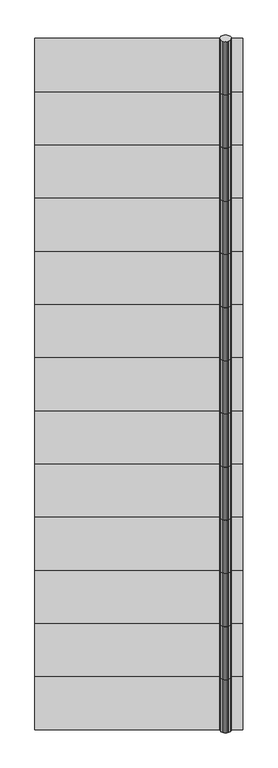
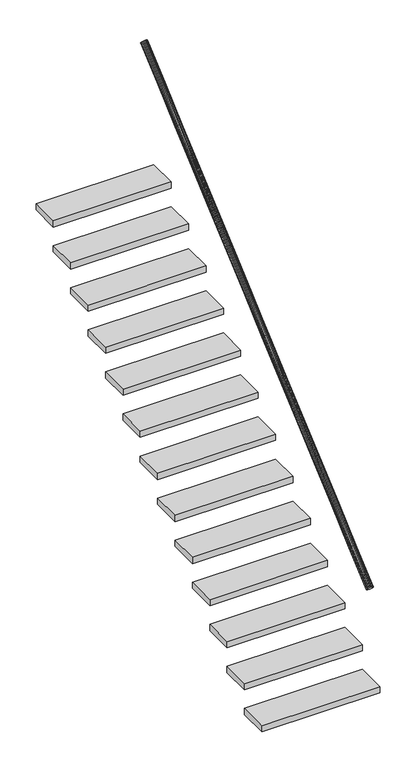
"""IFC4 building model written with IfcOpenShell, lengths in millimetres: stair geometry, 0_3d."""

from ifc_helpers import new_model, si_unit, frame, origin, origin_with_axes, place, context, project, spatial, polyline, outline, extrude, source, transform, mapped, element, save


def stair_800c35a0(model_context):
    return source(origin(), model_context, "Body", "SweptSolid", [
        extrude(outline(polyline([(900.0, 1165.003504), (0.0, 1165.003504), (0.0, 1395.003504), (900.0, 1395.003504), (900.0, 1165.003504)])), frame((0.0, 0.0, 1000.0), z_axis=(0.0, 0.0, 1.0), x_axis=(1.0, 0.0, 0.0)), (0.0, 0.0, 1.0), 50.0),
        extrude(outline(polyline([(900.0, 245.003504), (0.0, 245.003504), (0.0, 475.003504), (900.0, 475.003504), (900.0, 245.003504)])), frame((0.0, 0.0, 200.0), z_axis=(0.0, 0.0, 1.0), x_axis=(1.0, 0.0, 0.0)), (0.0, 0.0, 1.0), 50.0),
        extrude(outline(polyline([(1.2235871, -7.0656631), (0.0, 0.0), (1.2235871, 7.065663), (4.7745751, 13.4396897), (10.3053687, 18.4981459), (17.2745751, 21.7458748), (25.0, 22.8649659), (32.7254249, 21.7458748), (39.6946313, 18.4981459), (45.2254249, 13.4396897), (48.7764129, 7.065663), (50.0, 0.0), (48.7764129, -7.0656631), (45.2254249, -13.4396898), (39.6946313, -18.498146), (32.7254249, -21.7458748), (25.0, -22.864966), (17.2745751, -21.7458748), (10.3053687, -18.498146), (4.7745751, -13.4396898), (1.2235871, -7.0656631)])), frame((800.0, 1165.003504, 1869.5592366), z_axis=(0.0, 0.7546055221634054, 0.656178714924901), x_axis=(1.0, 0.0, 0.0)), (0.0, 0.0, 1.0), 304.7950131),
        extrude(outline(polyline([(1.2235871, -7.0656631), (0.0, 0.0), (1.2235871, 7.065663), (4.7745751, 13.4396897), (10.3053687, 18.4981459), (17.2745751, 21.7458748), (25.0, 22.8649659), (32.7254249, 21.7458748), (39.6946313, 18.4981459), (45.2254249, 13.4396897), (48.7764129, 7.065663), (50.0, 0.0), (48.7764129, -7.0656631), (45.2254249, -13.4396898), (39.6946313, -18.498146), (32.7254249, -21.7458748), (25.0, -22.864966), (17.2745751, -21.7458748), (10.3053687, -18.498146), (4.7745751, -13.4396898), (1.2235871, -7.0656631)])), frame((800.0, 475.003504, 1269.5592366), z_axis=(0.0, 0.7546055221634524, 0.6561787149248467), x_axis=(1.0, 0.0, 0.0)), (0.0, 0.0, 1.0), 304.7950131),
        extrude(outline(polyline([(1.2235871, -7.0656631), (0.0, 0.0), (1.2235871, 7.065663), (4.7745751, 13.4396897), (10.3053687, 18.4981459), (17.2745751, 21.7458748), (25.0, 22.8649659), (32.7254249, 21.7458748), (39.6946313, 18.4981459), (45.2254249, 13.4396897), (48.7764129, 7.065663), (50.0, 0.0), (48.7764129, -7.0656631), (45.2254249, -13.4396898), (39.6946313, -18.498146), (32.7254249, -21.7458748), (25.0, -22.864966), (17.2745751, -21.7458748), (10.3053687, -18.498146), (4.7745751, -13.4396898), (1.2235871, -7.0656631)])), frame((800.0, 2315.003504, 2869.5592366), z_axis=(0.0, 0.7546055221634114, 0.656178714924894), x_axis=(1.0, 0.0, 0.0)), (0.0, 0.0, 1.0), 304.7950131),
        extrude(outline(polyline([(1.2235871, -7.0656631), (0.0, 0.0), (1.2235871, 7.065663), (4.7745751, 13.4396897), (10.3053687, 18.4981459), (17.2745751, 21.7458748), (25.0, 22.8649659), (32.7254249, 21.7458748), (39.6946313, 18.4981459), (45.2254249, 13.4396897), (48.7764129, 7.065663), (50.0, 0.0), (48.7764129, -7.0656631), (45.2254249, -13.4396898), (39.6946313, -18.498146), (32.7254249, -21.7458748), (25.0, -22.864966), (17.2745751, -21.7458748), (10.3053687, -18.498146), (4.7745751, -13.4396898), (1.2235871, -7.0656631)])), frame((800.0, 705.003504, 1469.5592366), z_axis=(0.0, 0.7546055221634539, 0.656178714924845), x_axis=(1.0, 0.0, 0.0)), (0.0, 0.0, 1.0), 304.7950131),
        extrude(outline(polyline([(900.0, 2545.003504), (0.0, 2545.003504), (0.0, 2775.003504), (900.0, 2775.003504), (900.0, 2545.003504)])), frame((0.0, 0.0, 2200.0), z_axis=(0.0, 0.0, 1.0), x_axis=(1.0, 0.0, 0.0)), (0.0, 0.0, 1.0), 50.0),
        extrude(outline(polyline([(1.2235871, -7.0656631), (0.0, 0.0), (1.2235871, 7.065663), (4.7745751, 13.4396897), (10.3053687, 18.4981459), (17.2745751, 21.7458748), (25.0, 22.8649659), (32.7254249, 21.7458748), (39.6946313, 18.4981459), (45.2254249, 13.4396897), (48.7764129, 7.065663), (50.0, 0.0), (48.7764129, -7.0656631), (45.2254249, -13.4396898), (39.6946313, -18.498146), (32.7254249, -21.7458748), (25.0, -22.864966), (17.2745751, -21.7458748), (10.3053687, -18.498146), (4.7745751, -13.4396898), (1.2235871, -7.0656631)])), frame((800.0, 245.003504, 1069.5592366), z_axis=(0.0, 0.7546055221634513, 0.656178714924848), x_axis=(1.0, 0.0, 0.0)), (0.0, 0.0, 1.0), 304.7950131),
        extrude(outline(polyline([(1.2235871, -7.0656631), (0.0, 0.0), (1.2235871, 7.065663), (4.7745751, 13.4396897), (10.3053687, 18.4981459), (17.2745751, 21.7458748), (25.0, 22.8649659), (32.7254249, 21.7458748), (39.6946313, 18.4981459), (45.2254249, 13.4396897), (48.7764129, 7.065663), (50.0, 0.0), (48.7764129, -7.0656631), (45.2254249, -13.4396898), (39.6946313, -18.498146), (32.7254249, -21.7458748), (25.0, -22.864966), (17.2745751, -21.7458748), (10.3053687, -18.498146), (4.7745751, -13.4396898), (1.2235871, -7.0656631)])), frame((800.0, 2775.003504, 3269.5592366), z_axis=(0.0, 0.7546055221634004, 0.6561787149249065), x_axis=(1.0, 0.0, 0.0)), (0.0, 0.0, 1.0), 304.7950131),
        extrude(outline(polyline([(1.2235871, -7.0656631), (0.0, 0.0), (1.2235871, 7.065663), (4.7745751, 13.4396897), (10.3053687, 18.4981459), (17.2745751, 21.7458748), (25.0, 22.8649659), (32.7254249, 21.7458748), (39.6946313, 18.4981459), (45.2254249, 13.4396897), (48.7764129, 7.065663), (50.0, 0.0), (48.7764129, -7.0656631), (45.2254249, -13.4396898), (39.6946313, -18.498146), (32.7254249, -21.7458748), (25.0, -22.864966), (17.2745751, -21.7458748), (10.3053687, -18.498146), (4.7745751, -13.4396898), (1.2235871, -7.0656631)])), frame((800.0, 15.003504, 869.5592366), z_axis=(0.0, 0.7546055221634687, 0.6561787149248283), x_axis=(1.0, 0.0, 0.0)), (0.0, 0.0, 1.0), 304.7950131),
        extrude(outline(polyline([(900.0, 475.003504), (0.0, 475.003504), (0.0, 705.003504), (900.0, 705.003504), (900.0, 475.003504)])), frame((0.0, 0.0, 400.0), z_axis=(0.0, 0.0, 1.0), x_axis=(1.0, 0.0, 0.0)), (0.0, 0.0, 1.0), 50.0),
        extrude(outline(polyline([(1.2235871, -7.0656631), (0.0, 0.0), (1.2235871, 7.065663), (4.7745751, 13.4396897), (10.3053687, 18.4981459), (17.2745751, 21.7458748), (25.0, 22.8649659), (32.7254249, 21.7458748), (39.6946313, 18.4981459), (45.2254249, 13.4396897), (48.7764129, 7.065663), (50.0, 0.0), (48.7764129, -7.0656631), (45.2254249, -13.4396898), (39.6946313, -18.498146), (32.7254249, -21.7458748), (25.0, -22.864966), (17.2745751, -21.7458748), (10.3053687, -18.498146), (4.7745751, -13.4396898), (1.2235871, -7.0656631)])), frame((800.0, 1625.003504, 2269.5592366), z_axis=(0.0, 0.7546055221634052, 0.6561787149249012), x_axis=(1.0, 0.0, 0.0)), (0.0, 0.0, 1.0), 304.7950131),
        extrude(outline(polyline([(1.2235871, -7.0656631), (0.0, 0.0), (1.2235871, 7.065663), (4.7745751, 13.4396897), (10.3053687, 18.4981459), (17.2745751, 21.7458748), (25.0, 22.8649659), (32.7254249, 21.7458748), (39.6946313, 18.4981459), (45.2254249, 13.4396897), (48.7764129, 7.065663), (50.0, 0.0), (48.7764129, -7.0656631), (45.2254249, -13.4396898), (39.6946313, -18.498146), (32.7254249, -21.7458748), (25.0, -22.864966), (17.2745751, -21.7458748), (10.3053687, -18.498146), (4.7745751, -13.4396898), (1.2235871, -7.0656631)])), frame((800.0, 2545.003504, 3069.5592366), z_axis=(0.0, 0.7546055221634068, 0.6561787149248993), x_axis=(1.0, 0.0, 0.0)), (0.0, 0.0, 1.0), 304.7950131),
        extrude(outline(polyline([(900.0, 1395.003504), (0.0, 1395.003504), (0.0, 1625.003504), (900.0, 1625.003504), (900.0, 1395.003504)])), frame((0.0, 0.0, 1200.0), z_axis=(0.0, 0.0, 1.0), x_axis=(1.0, 0.0, 0.0)), (0.0, 0.0, 1.0), 50.0),
        extrude(outline(polyline([(900.0, 1855.003504), (0.0, 1855.003504), (0.0, 2085.003504), (900.0, 2085.003504), (900.0, 1855.003504)])), frame((0.0, 0.0, 1600.0), z_axis=(0.0, 0.0, 1.0), x_axis=(1.0, 0.0, 0.0)), (0.0, 0.0, 1.0), 50.0),
        extrude(outline(polyline([(1.2235871, -7.0656631), (0.0, 0.0), (1.2235871, 7.065663), (4.7745751, 13.4396897), (10.3053687, 18.4981459), (17.2745751, 21.7458748), (25.0, 22.8649659), (32.7254249, 21.7458748), (39.6946313, 18.4981459), (45.2254249, 13.4396897), (48.7764129, 7.065663), (50.0, 0.0), (48.7764129, -7.0656631), (45.2254249, -13.4396898), (39.6946313, -18.498146), (32.7254249, -21.7458748), (25.0, -22.864966), (17.2745751, -21.7458748), (10.3053687, -18.498146), (4.7745751, -13.4396898), (1.2235871, -7.0656631)])), frame((800.0, 1395.003504, 2069.5592366), z_axis=(0.0, 0.7546055221634034, 0.6561787149249032), x_axis=(1.0, 0.0, 0.0)), (0.0, 0.0, 1.0), 304.7950131),
        extrude(outline(polyline([(900.0, 935.003504), (0.0, 935.003504), (0.0, 1165.003504), (900.0, 1165.003504), (900.0, 935.003504)])), frame((0.0, 0.0, 800.0), z_axis=(0.0, 0.0, 1.0), x_axis=(1.0, 0.0, 0.0)), (0.0, 0.0, 1.0), 50.0),
        extrude(outline(polyline([(900.0, 705.003504), (0.0, 705.003504), (0.0, 935.003504), (900.0, 935.003504), (900.0, 705.003504)])), frame((0.0, 0.0, 600.0), z_axis=(0.0, 0.0, 1.0), x_axis=(1.0, 0.0, 0.0)), (0.0, 0.0, 1.0), 50.0),
        extrude(outline(polyline([(1.2235871, -7.0656631), (0.0, 0.0), (1.2235871, 7.065663), (4.7745751, 13.4396897), (10.3053687, 18.4981459), (17.2745751, 21.7458748), (25.0, 22.8649659), (32.7254249, 21.7458748), (39.6946313, 18.4981459), (45.2254249, 13.4396897), (48.7764129, 7.065663), (50.0, 0.0), (48.7764129, -7.0656631), (45.2254249, -13.4396898), (39.6946313, -18.498146), (32.7254249, -21.7458748), (25.0, -22.864966), (17.2745751, -21.7458748), (10.3053687, -18.498146), (4.7745751, -13.4396898), (1.2235871, -7.0656631)])), frame((800.0, 935.003504, 1669.5592366), z_axis=(0.0, 0.7546055221634518, 0.6561787149248475), x_axis=(1.0, 0.0, 0.0)), (0.0, 0.0, 1.0), 304.7950131),
        extrude(outline(polyline([(900.0, 2085.003504), (0.0, 2085.003504), (0.0, 2315.003504), (900.0, 2315.003504), (900.0, 2085.003504)])), frame((0.0, 0.0, 1800.0), z_axis=(0.0, 0.0, 1.0), x_axis=(1.0, 0.0, 0.0)), (0.0, 0.0, 1.0), 50.0),
        extrude(outline(polyline([(900.0, 2315.003504), (0.0, 2315.003504), (0.0, 2545.003504), (900.0, 2545.003504), (900.0, 2315.003504)])), frame((0.0, 0.0, 2000.0), z_axis=(0.0, 0.0, 1.0), x_axis=(1.0, 0.0, 0.0)), (0.0, 0.0, 1.0), 50.0),
        extrude(outline(polyline([(900.0, 2775.003504), (0.0, 2775.003504), (0.0, 3005.003504), (900.0, 3005.003504), (900.0, 2775.003504)])), frame((0.0, 0.0, 2400.0), z_axis=(0.0, 0.0, 1.0), x_axis=(1.0, 0.0, 0.0)), (0.0, 0.0, 1.0), 50.0),
        extrude(outline(polyline([(900.0, 1625.003504), (0.0, 1625.003504), (0.0, 1855.003504), (900.0, 1855.003504), (900.0, 1625.003504)])), frame((0.0, 0.0, 1400.0), z_axis=(0.0, 0.0, 1.0), x_axis=(1.0, 0.0, 0.0)), (0.0, 0.0, 1.0), 50.0),
        extrude(outline(polyline([(900.0, 15.003504), (0.0, 15.003504), (0.0, 245.003504), (900.0, 245.003504), (900.0, 15.003504)])), origin_with_axes(), (0.0, 0.0, 1.0), 50.0),
        extrude(outline(polyline([(1.2235871, -7.0656631), (0.0, 0.0), (1.2235871, 7.065663), (4.7745751, 13.4396897), (10.3053687, 18.4981459), (17.2745751, 21.7458748), (25.0, 22.8649659), (32.7254249, 21.7458748), (39.6946313, 18.4981459), (45.2254249, 13.4396897), (48.7764129, 7.065663), (50.0, 0.0), (48.7764129, -7.0656631), (45.2254249, -13.4396898), (39.6946313, -18.498146), (32.7254249, -21.7458748), (25.0, -22.864966), (17.2745751, -21.7458748), (10.3053687, -18.498146), (4.7745751, -13.4396898), (1.2235871, -7.0656631)])), frame((800.0, 1855.003504, 2469.5592366), z_axis=(0.0, 0.7546055221634105, 0.656178714924895), x_axis=(1.0, 0.0, 0.0)), (0.0, 0.0, 1.0), 304.7950131),
        extrude(outline(polyline([(1.2235871, -7.0656631), (0.0, 0.0), (1.2235871, 7.065663), (4.7745751, 13.4396897), (10.3053687, 18.4981459), (17.2745751, 21.7458748), (25.0, 22.8649659), (32.7254249, 21.7458748), (39.6946313, 18.4981459), (45.2254249, 13.4396897), (48.7764129, 7.065663), (50.0, 0.0), (48.7764129, -7.0656631), (45.2254249, -13.4396898), (39.6946313, -18.498146), (32.7254249, -21.7458748), (25.0, -22.864966), (17.2745751, -21.7458748), (10.3053687, -18.498146), (4.7745751, -13.4396898), (1.2235871, -7.0656631)])), frame((800.0, 2085.003504, 2669.5592366), z_axis=(0.0, 0.754605522163405, 0.6561787149249012), x_axis=(1.0, 0.0, 0.0)), (0.0, 0.0, 1.0), 304.7950131),
    ])


if __name__ == "__main__":
    model = new_model("IFC4")
    model_context = context("Model", 3, world=origin())
    ifc_project = project(units=[si_unit("LENGTHUNIT", "METRE", prefix="MILLI")], contexts=[model_context])
    site = spatial("IfcSite", under=ifc_project)
    building = spatial("IfcBuilding", under=site)
    placement = place(None, origin())
    stair_shape = stair_800c35a0(model_context)
    element("IfcStair", 1, ObjectType="0_3d", at=placement, inside=building, context=model_context, shape_type="MappedRepresentation", body=[
        mapped(stair_shape, transform((0.0, 0.0, 0.0), x_axis=(1.0, 0.0, 0.0), y_axis=(0.0, 1.0, 0.0), z_axis=(0.0, 0.0, 1.0))),
    ])
    save(model, "model.ifc")

# Revit data of these elements
# Element 1 (IfcStair, "0_3d")
#   Materials on its faces: "*1", "weiss"
# Materials
#   "*1": class "Unassigned", colour RGB 175 175 175, transparency 0
#   "weiss": class "Unassigned", colour RGB 255 255 255, transparency 0
